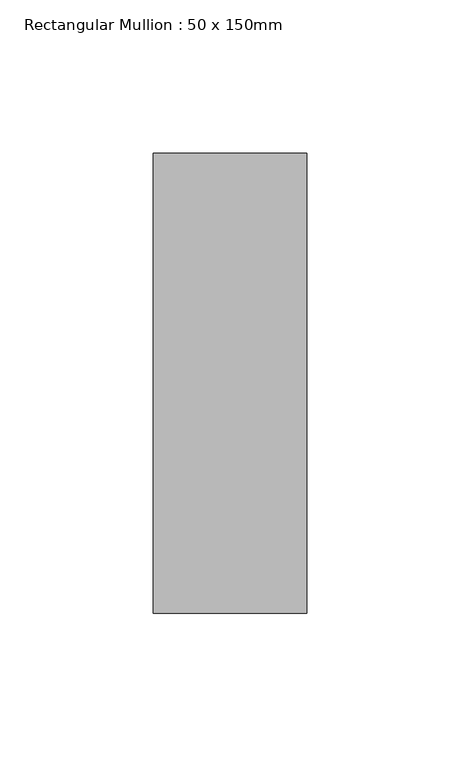
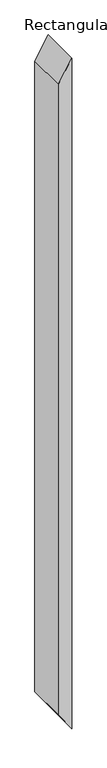
"""IFC4 building model written with IfcOpenShell, lengths in millimetres: member geometry, Rectangular Mullion : 50 x 150mm."""

from ifc_helpers import new_model, si_unit, frame, origin, place, context, project, spatial, polyline, outline, extrude, source, transform, mapped, element, save


def rectangular_mullion_50_x_150mm_faae0562(model_context):
    return source(origin(), model_context, "Body", "SweptSolid", [
        extrude(outline(polyline([(0.0, 0.0), (-85.321119, -50.0), (-2553.6011295, -50.0), (-2625.2230034, 0.0), (0.0, 0.0)])), frame((0.0, -75.0, 0.0), z_axis=(0.0, 1.0, 0.0), x_axis=(0.0, 0.0, 1.0)), (0.0, 0.0, 1.0), 150.0),
    ])


if __name__ == "__main__":
    model = new_model("IFC4")
    model_context = context("Model", 3, world=origin())
    ifc_project = project(units=[si_unit("LENGTHUNIT", "METRE", prefix="MILLI")], contexts=[model_context])
    site = spatial("IfcSite", under=ifc_project)
    building = spatial("IfcBuilding", under=site)
    placement = place(None, origin())
    rectangular_mullion_50_x_150mm_shape = rectangular_mullion_50_x_150mm_faae0562(model_context)
    element("IfcMember", 1, ObjectType="Rectangular Mullion : 50 x 150mm", at=placement, inside=building, context=model_context, shape_type="MappedRepresentation", body=[
        mapped(rectangular_mullion_50_x_150mm_shape, transform((0.0, 0.0, 0.0), x_axis=(1.0, 0.0, 0.0), y_axis=(0.0, 1.0, 0.0), z_axis=(0.0, 0.0, 1.0))),
    ])
    save(model, "model.ifc")

# Revit data of these elements
# Type "Rectangular Mullion : 50 x 150mm"
#   built-in parameter 1007304 = 0.492126 (stored number, unit not read)
#   built-in parameter 1007301 = 0.082021 (stored number, unit not read)
#   built-in parameter 1007300 = 0.082021 (stored number, unit not read)
# Element 1 (IfcMember, "Rectangular Mullion : 50 x 150mm")
#   Materials on its faces: "Metal - Aluminium"
# Materials
#   "Metal - Aluminium": class "Metal", colour RGB 247 247 247, transparency 0
